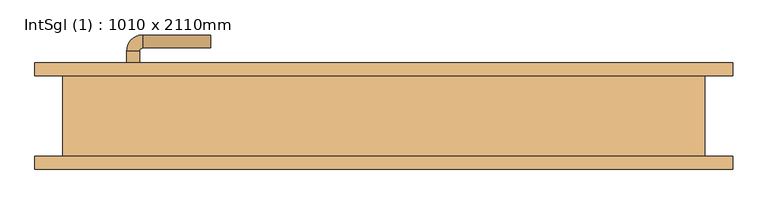
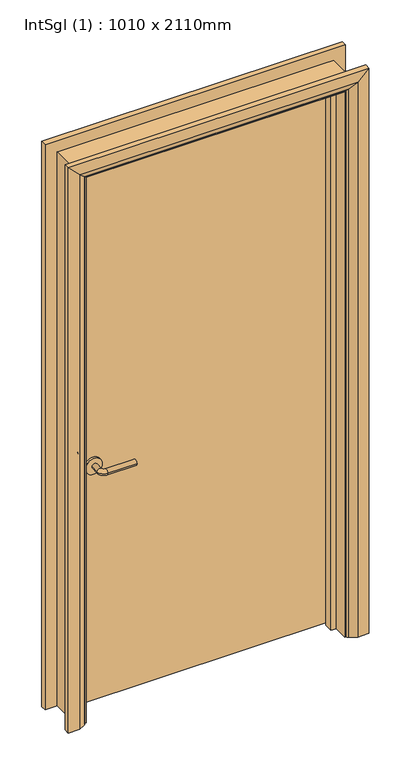
"""IFC4 building model written with IfcOpenShell, lengths in millimetres: door geometry, IntSgl (1) : 1010 x 2110mm."""

from ifc_helpers import new_model, si_unit, point, frame, frame_2d, origin, place, context, project, spatial, polyline, circle_curve, ellipse_curve, trimmed, segment, composite_curve, outline, extrude, faceted_brep, source, transform, mapped, element, save
from ifc_brep_helpers import plane_surface, cylinder_surface, revolved_surface, advanced_brep


def intsgl_1_1010_x_2110mm_2c20d0f1(model_context):
    return source(origin(), model_context, "Body", "SolidModel", [
        advanced_brep(
        [(-398.0, 16.5, 900.0), (-378.0, 16.5, 900.0), (-378.0, -13.5, 900.0), (-398.0, -13.5, 900.0), (-373.0, -18.5, 900.0), (-373.0, -38.5, 900.0), (-268.0, -38.5, 900.0), (-268.0, -18.5, 900.0)],
        [
            (0, 1, circle_curve(frame((-388.0, 16.5, 900.0), z_axis=(0.0, 1.0, 0.0), x_axis=(1.0, 0.0, 0.0)), 10.0)),
            (1, 0, circle_curve(frame((-388.0, 16.5, 900.0), z_axis=(0.0, 1.0, 0.0), x_axis=(1.0, 0.0, 0.0)), 10.0)),
            (1, 2),
            (2, 3, circle_curve(frame((-388.0, -13.5, 900.0), z_axis=(0.0, 1.0, 0.0), x_axis=(1.0, 0.0, 0.0)), 10.0)),
            (3, 0),
            (3, 2, circle_curve(frame((-388.0, -13.5, 900.0), z_axis=(0.0, 1.0, 0.0), x_axis=(1.0, 0.0, 0.0)), 10.0)),
            (4, 5, circle_curve(frame((-373.0, -28.5, 900.0), z_axis=(-1.0, 0.0, 0.0), x_axis=(0.0, 1.0, 0.0)), 10.0)),
            (5, 3, circle_curve(frame((-373.0, -13.5, 900.0), z_axis=(0.0, 0.0, -1.0), x_axis=(-1.0, 0.0, 0.0)), 25.0)),
            (2, 4, circle_curve(frame((-373.0, -13.5, 900.0), z_axis=(0.0, 0.0, 1.0), x_axis=(-1.0, 0.0, 0.0)), 5.0)),
            (5, 4, circle_curve(frame((-373.0, -28.5, 900.0), z_axis=(-1.0, 0.0, 0.0), x_axis=(0.0, 1.0, 0.0)), 10.0)),
            (6, 7, circle_curve(frame((-268.0, -28.5, 900.0), z_axis=(1.0, 0.0, 0.0), x_axis=(0.0, 1.0, 0.0)), 10.0)),
            (7, 6, circle_curve(frame((-268.0, -28.5, 900.0), z_axis=(1.0, 0.0, 0.0), x_axis=(0.0, 1.0, 0.0)), 10.0)),
            (4, 7),
            (6, 5),
        ],
        [
            plane_surface(frame((-388.0, 16.5, 900.0), z_axis=(0.0, 1.0, 0.0), x_axis=(0.0, 0.0, 1.0))),
            cylinder_surface(frame((-388.0, 16.5, 900.0), z_axis=(0.0, 1.0, 0.0), x_axis=(1.0, 0.0, 0.0)), 10.0),
            revolved_surface(trimmed(ellipse_curve(frame((-388.0, -13.5, 900.0), z_axis=(0.0, -1.0, 0.0), x_axis=(1.0, 0.0, 0.0)), 10.0, 10.0), [point((-398.0, -13.5, 900.0))], [point((-378.0, -13.5, 900.0))], True, "CARTESIAN"), (-373.0, -13.5, 900.0), (0.0, 0.0, -1.0)),
            revolved_surface(trimmed(ellipse_curve(frame((-388.0, -13.5, 900.0), z_axis=(0.0, -1.0, 0.0), x_axis=(1.0, 0.0, 0.0)), 10.0, 10.0), [point((-378.0, -13.5, 900.0))], [point((-398.0, -13.5, 900.0))], True, "CARTESIAN"), (-373.0, -13.5, 900.0), (0.0, 0.0, -1.0)),
            plane_surface(frame((-268.0, -28.5, 900.0), z_axis=(1.0, 0.0, 0.0), x_axis=(0.0, 0.0, 1.0))),
            cylinder_surface(frame((-373.0, -28.5, 900.0), z_axis=(-1.0, 0.0, 0.0), x_axis=(0.0, 1.0, 0.0)), 10.0),
        ],
        [
            (0, [[1, 2]]),
            (1, [[3, 4, 5, -2]]),
            (1, [[-5, 6, -3, -1]]),
            (2, [[7, 8, -4, 9]]),
            (3, [[10, -9, -6, -8]]),
            (4, [[11, 12]]),
            (5, [[13, -11, 14, -7]]),
            (5, [[-14, -12, -13, -10]]),
        ],
    ),
        extrude(outline(composite_curve([segment(trimmed(circle_curve(frame_2d((900.0, -390.5)), 30.0), [point((900.0, -420.5))], [point((900.0, -360.5))], False, "CARTESIAN"), True, "CONTINUOUS"), segment(trimmed(circle_curve(frame_2d((900.0, -390.5)), 30.0), [point((900.0, -360.5))], [point((900.0, -420.5))], False, "CARTESIAN"), True, "CONTINUOUS")], self_intersect=False)), frame((0.0, 16.5, 0.0), z_axis=(0.0, 1.0, 0.0), x_axis=(0.0, 0.0, 1.0)), (0.0, 0.0, 1.0), 8.0),
        advanced_brep(
        [(-398.0, 70.5, 900.0), (-378.0, 70.5, 900.0), (-398.0, 100.5, 900.0), (-378.0, 100.5, 900.0), (-373.0, 105.5, 900.0), (-373.0, 125.5, 900.0), (-268.0, 125.5, 900.0), (-268.0, 105.5, 900.0)],
        [
            (0, 1, circle_curve(frame((-388.0, 70.5, 900.0), z_axis=(0.0, -1.0, 0.0), x_axis=(1.0, 0.0, 0.0)), 10.0)),
            (1, 0, circle_curve(frame((-388.0, 70.5, 900.0), z_axis=(0.0, -1.0, 0.0), x_axis=(1.0, 0.0, 0.0)), 10.0)),
            (0, 2),
            (2, 3, circle_curve(frame((-388.0, 100.5, 900.0), z_axis=(0.0, -1.0, 0.0), x_axis=(1.0, 0.0, 0.0)), 10.0)),
            (3, 1),
            (3, 2, circle_curve(frame((-388.0, 100.5, 900.0), z_axis=(0.0, -1.0, 0.0), x_axis=(1.0, 0.0, 0.0)), 10.0)),
            (4, 3, circle_curve(frame((-373.0, 100.5, 900.0), z_axis=(0.0, 0.0, 1.0), x_axis=(-1.0, 0.0, 0.0)), 5.0)),
            (2, 5, circle_curve(frame((-373.0, 100.5, 900.0), z_axis=(0.0, 0.0, -1.0), x_axis=(-1.0, 0.0, 0.0)), 25.0)),
            (5, 4, circle_curve(frame((-373.0, 115.5, 900.0), z_axis=(-1.0, 0.0, 0.0), x_axis=(0.0, -1.0, 0.0)), 10.0)),
            (4, 5, circle_curve(frame((-373.0, 115.5, 900.0), z_axis=(-1.0, 0.0, 0.0), x_axis=(0.0, -1.0, 0.0)), 10.0)),
            (6, 7, circle_curve(frame((-268.0, 115.5, 900.0), z_axis=(1.0, 0.0, 0.0), x_axis=(0.0, -1.0, 0.0)), 10.0)),
            (7, 6, circle_curve(frame((-268.0, 115.5, 900.0), z_axis=(1.0, 0.0, 0.0), x_axis=(0.0, -1.0, 0.0)), 10.0)),
            (5, 6),
            (7, 4),
        ],
        [
            plane_surface(frame((-388.0, 70.5, 900.0), z_axis=(0.0, -1.0, 0.0), x_axis=(0.0, 0.0, 1.0))),
            cylinder_surface(frame((-388.0, 70.5, 900.0), z_axis=(0.0, -1.0, 0.0), x_axis=(1.0, 0.0, 0.0)), 10.0),
            revolved_surface(trimmed(ellipse_curve(frame((-388.0, 100.5, 900.0), z_axis=(0.0, -1.0, 0.0), x_axis=(1.0, 0.0, 0.0)), 10.0, 10.0), [point((-398.0, 100.5, 900.0))], [point((-378.0, 100.5, 900.0))], True, "CARTESIAN"), (-373.0, 100.5, 900.0), (0.0, 0.0, -1.0)),
            revolved_surface(trimmed(ellipse_curve(frame((-388.0, 100.5, 900.0), z_axis=(0.0, -1.0, 0.0), x_axis=(1.0, 0.0, 0.0)), 10.0, 10.0), [point((-378.0, 100.5, 900.0))], [point((-398.0, 100.5, 900.0))], True, "CARTESIAN"), (-373.0, 100.5, 900.0), (0.0, 0.0, -1.0)),
            plane_surface(frame((-268.0, 115.5, 900.0), z_axis=(1.0, 0.0, 0.0), x_axis=(0.0, 0.0, 1.0))),
            cylinder_surface(frame((-373.0, 115.5, 900.0), z_axis=(-1.0, 0.0, 0.0), x_axis=(0.0, -1.0, 0.0)), 10.0),
        ],
        [
            (0, [[1, 2]]),
            (1, [[-1, 3, 4, 5]]),
            (1, [[-2, -5, 6, -3]]),
            (2, [[7, -4, 8, 9]]),
            (3, [[-8, -6, -7, 10]]),
            (4, [[11, 12]]),
            (5, [[-9, 13, -12, 14]]),
            (5, [[-10, -14, -11, -13]]),
        ],
    ),
        extrude(outline(composite_curve([segment(trimmed(circle_curve(frame_2d((900.0, -390.5)), 30.0), [point((900.0, -420.5))], [point((900.0, -360.5))], False, "CARTESIAN"), True, "CONTINUOUS"), segment(trimmed(circle_curve(frame_2d((900.0, -390.5)), 30.0), [point((900.0, -360.5))], [point((900.0, -420.5))], False, "CARTESIAN"), True, "CONTINUOUS")], self_intersect=False)), frame((0.0, 62.5, 0.0), z_axis=(0.0, 1.0, 0.0), x_axis=(0.0, 0.0, 1.0)), (0.0, 0.0, 1.0), 8.0),
        extrude(outline(polyline([(463.0, 24.5), (-463.0, 24.5), (-463.0, 62.5), (463.0, 62.5), (463.0, 24.5)])), frame((0.0, 0.0, 8.0), z_axis=(0.0, 0.0, 1.0), x_axis=(1.0, 0.0, 0.0)), (0.0, 0.0, 1.0), 2060.0),
        advanced_brep(
        [(540.0, 82.5, 0.0), (540.0, 62.5, 0.0), (470.0, 62.5, 0.0), (474.0, 68.5, 0.0), (500.0, 82.5, 0.0), (540.0, 82.5, 2145.0), (540.0, 62.5, 2145.0), (-540.0, 62.5, 2145.0), (-540.0, 62.5, 0.0), (-470.0, 62.5, 0.0), (-470.0, 62.5, 2075.0), (470.0, 62.5, 2075.0), (474.0, 68.5, 2079.0), (500.0, 82.5, 2105.0), (-500.0, 82.5, 2105.0), (-500.0, 82.5, 0.0), (-540.0, 82.5, 0.0), (-540.0, 82.5, 2145.0), (-474.0, 68.5, 2079.0), (-474.0, 68.5, 0.0)],
        [
            (0, 1),
            (1, 2),
            (2, 3, circle_curve(frame((478.0, 61.5, 0.0), z_axis=(0.0, 0.0, -1.0), x_axis=(1.0, 0.0, 0.0)), 8.0622577)),
            (3, 4),
            (4, 0),
            (0, 5),
            (5, 6),
            (6, 1),
            (6, 7),
            (7, 8),
            (8, 9),
            (9, 10),
            (10, 11),
            (11, 2),
            (11, 12, ellipse_curve(frame((478.0, 61.5, 2083.0), z_axis=(0.7071067811865475, 0.0, -0.7071067811865475), x_axis=(-0.7071067811865474, 0.0, -0.7071067811865476)), 11.4017543, 8.0622577)),
            (12, 3),
            (12, 13),
            (13, 4),
            (13, 14),
            (14, 15),
            (15, 16),
            (16, 17),
            (17, 5),
            (17, 7),
            (10, 18, ellipse_curve(frame((-478.0, 61.5, 2083.0), z_axis=(0.7071067811865475, 0.0, 0.7071067811865475), x_axis=(0.7071067811865476, 0.0, -0.7071067811865474)), 11.4017543, 8.0622577)),
            (18, 12),
            (18, 14),
            (15, 19),
            (19, 9, circle_curve(frame((-478.0, 61.5, 0.0), z_axis=(0.0, 0.0, -1.0), x_axis=(-1.0, 0.0, 0.0)), 8.0622577)),
            (8, 16),
            (19, 18),
        ],
        [
            plane_surface(frame((470.0, 62.5, 0.0), z_axis=(0.0, 0.0, -1.0), x_axis=(0.0, -1.0, 0.0))),
            plane_surface(frame((540.0, 82.5, 0.0), z_axis=(1.0, 0.0, 0.0), x_axis=(0.0, 0.0, 1.0))),
            plane_surface(frame((540.0, 62.5, 0.0), z_axis=(0.0, -1.0, 0.0), x_axis=(0.0, 0.0, 1.0))),
            cylinder_surface(frame((478.0, 61.5, 0.0), z_axis=(0.0, 0.0, -1.0), x_axis=(1.0, 0.0, 0.0)), 8.0622577),
            plane_surface(frame((474.0, 68.5, 0.0), z_axis=(-0.4740998230350126, 0.880471099922178, 0.0), x_axis=(0.0, 0.0, 1.0))),
            plane_surface(frame((500.0, 82.5, 0.0), z_axis=(0.0, 1.0, 0.0), x_axis=(0.0, 0.0, 1.0))),
            plane_surface(frame((540.0, 82.5, 2145.0), z_axis=(0.0, 0.0, 1.0), x_axis=(-1.0, 0.0, 0.0))),
            cylinder_surface(frame((470.0, 61.5, 2083.0), z_axis=(1.0, 0.0, 0.0), x_axis=(0.0, 0.0, 1.0)), 8.0622577),
            plane_surface(frame((474.0, 68.5, 2079.0), z_axis=(0.0, 0.8804710999221764, -0.4740998230350154), x_axis=(-1.0, 0.0, 0.0))),
            plane_surface(frame((-470.0, 62.5, 0.0), z_axis=(0.0, 0.0, -1.0), x_axis=(0.0, -1.0, 0.0))),
            plane_surface(frame((-540.0, 82.5, 2145.0), z_axis=(-1.0, 0.0, 0.0), x_axis=(0.0, 0.0, -1.0))),
            cylinder_surface(frame((-478.0, 61.5, 2075.0), z_axis=(0.0, 0.0, 1.0), x_axis=(-1.0, 0.0, 0.0)), 8.0622577),
            plane_surface(frame((-474.0, 68.5, 2079.0), z_axis=(0.47409982303501824, 0.8804710999221749, 0.0), x_axis=(0.0, 0.0, -1.0))),
        ],
        [
            (0, [[1, 2, 3, 4, 5]]),
            (1, [[-1, 6, 7, 8]]),
            (2, [[-2, -8, 9, 10, 11, 12, 13, 14]]),
            (3, [[-3, -14, 15, 16]]),
            (4, [[-4, -16, 17, 18]]),
            (5, [[-5, -18, 19, 20, 21, 22, 23, -6]]),
            (6, [[-7, -23, 24, -9]]),
            (7, [[-15, -13, 25, 26]]),
            (8, [[-17, -26, 27, -19]]),
            (9, [[-21, 28, 29, -11, 30]]),
            (10, [[-24, -22, -30, -10]]),
            (11, [[-25, -12, -29, 31]]),
            (12, [[-27, -31, -28, -20]]),
        ],
    ),
        extrude(outline(polyline([(0.0, -465.0), (0.0, -446.0), (2051.0, -446.0), (2051.0, 446.0), (0.0, 446.0), (0.0, 465.0), (2070.0, 465.0), (2070.0, -465.0), (0.0, -465.0)])), frame((0.0, -9.5, 0.0), z_axis=(0.0, 1.0, 0.0), x_axis=(0.0, 0.0, 1.0)), (0.0, 0.0, 1.0), 32.0),
        advanced_brep(
        [(-540.0, -82.5, 0.0), (-540.0, -62.5, 0.0), (-470.0, -62.5, 0.0), (-474.0, -68.5, 0.0), (-500.0, -82.5, 0.0), (-540.0, -82.5, 2145.0), (-540.0, -62.5, 2145.0), (-470.0, -62.5, 2075.0), (-474.0, -68.5, 2079.0), (-500.0, -82.5, 2105.0), (540.0, -82.5, 2145.0), (540.0, -62.5, 2145.0), (470.0, -62.5, 2075.0), (474.0, -68.5, 2079.0), (500.0, -82.5, 2105.0), (540.0, -82.5, 0.0), (500.0, -82.5, 0.0), (474.0, -68.5, 0.0), (470.0, -62.5, 0.0), (540.0, -62.5, 0.0)],
        [
            (0, 1),
            (1, 2),
            (2, 3, circle_curve(frame((-478.0, -61.5, 0.0), z_axis=(0.0, 0.0, -1.0), x_axis=(-1.0, 0.0, 0.0)), 8.0622577)),
            (3, 4),
            (4, 0),
            (0, 5),
            (5, 6),
            (6, 1),
            (6, 7),
            (7, 2),
            (7, 8, ellipse_curve(frame((-478.0, -61.5, 2083.0), z_axis=(-0.7071067811865475, 0.0, -0.7071067811865475), x_axis=(0.7071067811865474, 0.0, -0.7071067811865476)), 11.4017543, 8.0622577)),
            (8, 3),
            (8, 9),
            (9, 4),
            (9, 5),
            (5, 10),
            (10, 11),
            (11, 6),
            (11, 12),
            (12, 7),
            (12, 13, ellipse_curve(frame((478.0, -61.5, 2083.0), z_axis=(-0.7071067811865475, 0.0, 0.7071067811865475), x_axis=(-0.7071067811865476, 0.0, -0.7071067811865474)), 11.4017543, 8.0622577)),
            (13, 8),
            (13, 14),
            (14, 9),
            (14, 10),
            (15, 16),
            (16, 17),
            (17, 18, circle_curve(frame((478.0, -61.5, 0.0), z_axis=(0.0, 0.0, -1.0), x_axis=(1.0, 0.0, 0.0)), 8.0622577)),
            (18, 19),
            (19, 15),
            (10, 15),
            (19, 11),
            (18, 12),
            (17, 13),
            (16, 14),
        ],
        [
            plane_surface(frame((-470.0, -135.3010989, 0.0), z_axis=(0.0, 0.0, -1.0), x_axis=(1.0, 0.0, 0.0))),
            plane_surface(frame((-540.0, -82.5, 0.0), z_axis=(-1.0, 0.0, 0.0), x_axis=(0.0, 0.0, 1.0))),
            plane_surface(frame((-540.0, -62.5, 0.0), z_axis=(0.0, 1.0, 0.0), x_axis=(0.0, 0.0, 1.0))),
            cylinder_surface(frame((-478.0, -61.5, 0.0), z_axis=(0.0, 0.0, -1.0), x_axis=(-1.0, 0.0, 0.0)), 8.0622577),
            plane_surface(frame((-474.0, -68.5, 0.0), z_axis=(0.4740998230350183, -0.8804710999221749, 0.0), x_axis=(0.0, 0.0, 1.0))),
            plane_surface(frame((-500.0, -82.5, 0.0), z_axis=(0.0, -1.0, 0.0), x_axis=(0.0, 0.0, 1.0))),
            plane_surface(frame((-540.0, -82.5, 2145.0), z_axis=(0.0, 0.0, 1.0), x_axis=(1.0, 0.0, 0.0))),
            plane_surface(frame((-540.0, -62.5, 2145.0), z_axis=(0.0, 1.0, 0.0), x_axis=(1.0, 0.0, 0.0))),
            cylinder_surface(frame((-470.0, -61.5, 2083.0), z_axis=(-1.0, 0.0, 0.0), x_axis=(0.0, 0.0, 1.0)), 8.0622577),
            plane_surface(frame((-474.0, -68.5, 2079.0), z_axis=(0.0, -0.8804710999221749, -0.4740998230350183), x_axis=(1.0, 0.0, 0.0))),
            plane_surface(frame((-500.0, -82.5, 2105.0), z_axis=(0.0, -1.0, 0.0), x_axis=(1.0, 0.0, 0.0))),
            plane_surface(frame((470.0, -135.3010989, 0.0), z_axis=(0.0, 0.0, -1.0), x_axis=(-1.0, 0.0, 0.0))),
            plane_surface(frame((540.0, -82.5, 2145.0), z_axis=(1.0, 0.0, 0.0), x_axis=(0.0, 0.0, -1.0))),
            plane_surface(frame((540.0, -62.5, 2145.0), z_axis=(0.0, 1.0, 0.0), x_axis=(0.0, 0.0, -1.0))),
            cylinder_surface(frame((478.0, -61.5, 2075.0), z_axis=(0.0, 0.0, 1.0), x_axis=(1.0, 0.0, 0.0)), 8.0622577),
            plane_surface(frame((474.0, -68.5, 2079.0), z_axis=(-0.4740998230350183, -0.8804710999221749, 0.0), x_axis=(0.0, 0.0, -1.0))),
            plane_surface(frame((500.0, -82.5, 2105.0), z_axis=(0.0, -1.0, 0.0), x_axis=(0.0, 0.0, -1.0))),
        ],
        [
            (0, [[1, 2, 3, 4, 5]]),
            (1, [[-1, 6, 7, 8]]),
            (2, [[-2, -8, 9, 10]]),
            (3, [[-3, -10, 11, 12]]),
            (4, [[-4, -12, 13, 14]]),
            (5, [[-5, -14, 15, -6]]),
            (6, [[-7, 16, 17, 18]]),
            (7, [[-9, -18, 19, 20]]),
            (8, [[-11, -20, 21, 22]]),
            (9, [[-13, -22, 23, 24]]),
            (10, [[-15, -24, 25, -16]]),
            (11, [[26, 27, 28, 29, 30]]),
            (12, [[-17, 31, -30, 32]]),
            (13, [[-19, -32, -29, 33]]),
            (14, [[-21, -33, -28, 34]]),
            (15, [[-23, -34, -27, 35]]),
            (16, [[-25, -35, -26, -31]]),
        ],
    ),
        faceted_brep([(-465.0, 62.5, 0.0), (-465.0, -62.5, 0.0), (-497.0, -62.5, 0.0), (-497.0, 62.5, 0.0), (-465.0, 62.5, 2070.0), (-465.0, -62.5, 2070.0), (-497.0, -62.5, 2102.0), (-497.0, 62.5, 2102.0), (465.0, 62.5, 2070.0), (465.0, -62.5, 2070.0), (497.0, -62.5, 2102.0), (497.0, 62.5, 2102.0), (465.0, 62.5, 0.0), (497.0, 62.5, 0.0), (497.0, -62.5, 0.0), (465.0, -62.5, 0.0)], [[[0, 1, 2, 3]], [[1, 0, 4, 5]], [[2, 1, 5, 6]], [[3, 2, 6, 7]], [[0, 3, 7, 4]], [[5, 4, 8, 9]], [[6, 5, 9, 10]], [[7, 6, 10, 11]], [[4, 7, 11, 8]], [[12, 13, 14, 15]], [[9, 8, 12, 15]], [[10, 9, 15, 14]], [[11, 10, 14, 13]], [[8, 11, 13, 12]]]),
    ])


if __name__ == "__main__":
    model = new_model("IFC4")
    model_context = context("Model", 3, world=origin())
    ifc_project = project(units=[si_unit("LENGTHUNIT", "METRE", prefix="MILLI")], contexts=[model_context])
    site = spatial("IfcSite", under=ifc_project)
    building = spatial("IfcBuilding", under=site)
    placement = place(None, origin())
    intsgl_1_1010_x_2110mm_shape = intsgl_1_1010_x_2110mm_2c20d0f1(model_context)
    element("IfcDoor", 1, ObjectType="IntSgl (1) : 1010 x 2110mm", at=placement, inside=building, context=model_context, shape_type="MappedRepresentation", body=[
        mapped(intsgl_1_1010_x_2110mm_shape, transform((0.0, 0.0, 0.0), x_axis=(1.0, 0.0, 0.0), y_axis=(0.0, 1.0, 0.0), z_axis=(0.0, 0.0, 1.0))),
    ])
    save(model, "model.ifc")

# Revit data of these elements
# Type "IntSgl (1) : 1010 x 2110mm"
#   Construction Type Id = "MDOOR"
#   Analytic Construction = "Metal"
#   Type Mark = "43"
#   Type Comments = "Internal Single"
#   Operation = "SingleSwingRight"
#   Manufacturer = "Revit"
#   Keynote = "L20"
#   Description = "Internal Single Door"
#   Visual Light Transmittance = 0
#   Solar Heat Gain Coefficient = 0
#   Heat Transfer Coefficient (U) = 3.7021 W/(m²·K)
#   UnderCut = 8 mm
#   Tolerance = 2 mm
#   Thickness = 38 mm
#   Structural Tolerance = 8 mm
#   StopDepth = 32 mm
#   Stop Thickness = 19 mm
#   Rough Width = 1010 mm
#   Rough Height = 2110 mm
#   Height to Top Lock Rail = 1000 mm
#   Handle Z Distance = 900 mm
#   Handle X Distance = 75 mm
#   Frame Thickness = 32 mm
#   Door Panel Width = 926 mm
#   Door Panel Thickness = 38 mm
#   Door Panel Offset = 0 mm
#   Height = 2110 mm
#   Width = 1010 mm
#   Door Panel Height = 2060 mm
#   Architrave Setback = 5 mm
#   Function = 0
#   Vis - Ironmongery = yes
#   Material Ironmongery = Door - Handle
#   Material Frame = Door - Frame/Mullion (1)
#   Material Door = Door - Panel
#   Material Architrave = Door - Architrave
#   Wall Closure = (empty or 0)
# Element 1 (IfcDoor, "IntSgl (1) : 1010 x 2110mm")
#   Materials on its faces: "Door - Architrave", "Door - Handle", "Door - Frame/Mullion (1)", "Door - Panel"
# Materials
#   "Door - Handle": class "Miscellaneous", colour RGB 0 0 0, transparency 0, Keynote = "P21"
#   "Door - Frame/Mullion (1)": class "Wood", colour RGB 212 179 113, transparency 0, Keynote = "L20", Cost = 0
#   "Door - Panel": class "Wood", colour RGB 210 159 95, transparency 0, Keynote = "L20"
#   "Door - Architrave": class "Wood", colour RGB 154 90 5, transparency 0, Keynote = "P20"
